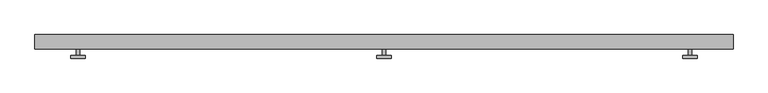
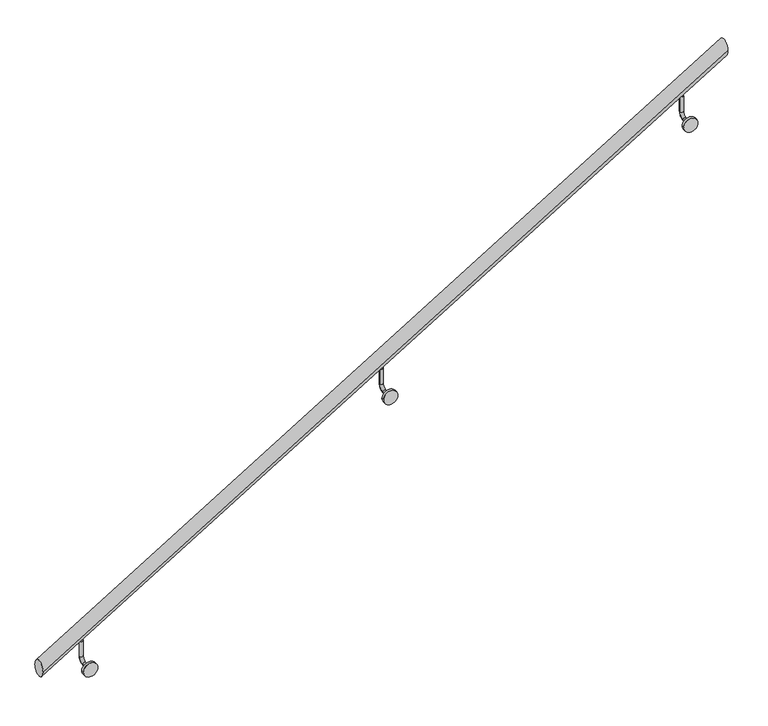
"""IFC4 building model written with IfcOpenShell, lengths in millimetres: railing geometry."""

import ifcopenshell
import ifcopenshell.guid

model = None  # the IFC model being written
_history = None  # IfcOwnerHistory: only IFC2X3 demands one
_inside = {}  # id of a spatial element -> (the spatial element, [elements in it])
_under = {}  # id of a project, library or spatial element -> (it, [spatial elements below it])
_declared = {}  # id of a project -> (the project, [libraries it declares])
_typed = {}  # id of a type object -> (the type object, [elements of that type])
_made_of = {}  # id of a material, layer set ... -> (it, [elements and type objects made of it])


def new_model(schema):
    """Start an empty IFC model of exactly this schema.

    Asked for "IFC4X3", IfcOpenShell would pick the latest addendum, in which some entities
    have other attributes; the version numbers below select the first issue.
    IFC2X3 requires an IfcOwnerHistory on every rooted entity: one is made here for all.
    """
    global model, _history
    if schema == "IFC4X3":
        model = ifcopenshell.file(schema_version=(4, 3, 0, 0))
    else:
        model = ifcopenshell.file(schema=schema)
    _inside.clear()
    _under.clear()
    _declared.clear()
    _typed.clear()
    _made_of.clear()
    _history = None
    if model.schema == "IFC2X3":
        org = make("IfcOrganization", Name="unknown")
        user = make(
            "IfcPersonAndOrganization",
            ThePerson=make("IfcPerson", FamilyName="unknown"),
            TheOrganization=org,
        )
        app = make(
            "IfcApplication",
            ApplicationDeveloper=org,
            Version="unknown",
            ApplicationFullName="unknown",
            ApplicationIdentifier="unknown",
        )
        _history = make(
            "IfcOwnerHistory",
            OwningUser=user,
            OwningApplication=app,
            ChangeAction="ADDED",
            CreationDate=0,
        )
    return model


def make(cls, **values):
    """One entity of the class cls with the attributes given. An attribute that is None is left unset."""
    return model.create_entity(
        cls, **{name: value for name, value in values.items() if value is not None}
    )


def rooted(cls, **values):
    """An entity with a GlobalId (a new one), such as an element, a storey or a relation."""
    return make(cls, GlobalId=ifcopenshell.guid.new(), OwnerHistory=_history, **values)


def si_unit(unit_type, name, prefix=None):
    """IfcSIUnit, for example si_unit("LENGTHUNIT", "METRE", prefix="MILLI")."""
    return make("IfcSIUnit", UnitType=unit_type, Prefix=prefix, Name=name)


def assignment(units):
    """IfcUnitAssignment: the units of a project."""
    return None if units is None else make("IfcUnitAssignment", Units=units)


def point(xyz):
    """IfcCartesianPoint."""
    return None if xyz is None else make("IfcCartesianPoint", Coordinates=xyz)


def direction(xyz):
    """IfcDirection."""
    return None if xyz is None else make("IfcDirection", DirectionRatios=xyz)


def frame(location, z_axis=None, x_axis=None):
    """IfcAxis2Placement3D, a coordinate frame: its origin and axes. An axis left out is left unset."""
    return make(
        "IfcAxis2Placement3D",
        Location=point(location),
        Axis=direction(z_axis),
        RefDirection=direction(x_axis),
    )


def frame_2d(location, x_axis=None):
    """IfcAxis2Placement2D, a coordinate frame in the plane: its origin and x axis."""
    return make(
        "IfcAxis2Placement2D", Location=point(location), RefDirection=direction(x_axis)
    )


def origin():
    """The frame at (0, 0, 0) with its axes left unset."""
    return frame((0.0, 0.0, 0.0))


def place(relative_to, where):
    """IfcLocalPlacement: puts the frame where relative to a parent placement (None: the world)."""
    return make(
        "IfcLocalPlacement", PlacementRelTo=relative_to, RelativePlacement=where
    )


def context(
    kind, dimensions, precision=None, world=None, true_north=None, identifier=None
):
    """IfcGeometricRepresentationContext, for example the 3D "Model" context."""
    return make(
        "IfcGeometricRepresentationContext",
        ContextIdentifier=identifier,
        ContextType=kind,
        CoordinateSpaceDimension=dimensions,
        Precision=precision,
        WorldCoordinateSystem=world,
        TrueNorth=true_north,
    )


def project(units=None, contexts=None):
    """IfcProject with its units and contexts."""
    return rooted(
        "IfcProject",
        Name="project",
        RepresentationContexts=contexts,
        UnitsInContext=assignment(units),
    )


def spatial(cls, under=None, at=None, **own):
    """A site, building, storey or space (cls), placed at a placement, below another one or the project."""
    s = rooted(cls, ObjectPlacement=at, **own)
    if under is not None:
        _under.setdefault(under.id(), (under, []))[1].append(s)
    return s


def circle_curve(where, radius):
    """IfcCircle in the frame where."""
    return make("IfcCircle", Position=where, Radius=radius)


def ellipse_curve(where, semi_axis1, semi_axis2):
    """IfcEllipse in the frame where."""
    return make(
        "IfcEllipse", Position=where, SemiAxis1=semi_axis1, SemiAxis2=semi_axis2
    )


def trimmed(basis, trim1, trim2, sense, master):
    """IfcTrimmedCurve: the piece of a basis curve between two trims."""
    return make(
        "IfcTrimmedCurve",
        BasisCurve=basis,
        Trim1=trim1,
        Trim2=trim2,
        SenseAgreement=sense,
        MasterRepresentation=master,
    )


def segment(curve, same_sense, transition):
    """IfcCompositeCurveSegment."""
    return make(
        "IfcCompositeCurveSegment",
        Transition=transition,
        SameSense=same_sense,
        ParentCurve=curve,
    )


def composite_curve(segments, self_intersect=None):
    """IfcCompositeCurve: segments joined end to end."""
    return make("IfcCompositeCurve", Segments=segments, SelfIntersect=self_intersect)


def outline(outer, holes=None, kind="AREA"):
    """IfcArbitraryClosedProfileDef: a profile drawn as a closed curve; with holes, ...WithVoids."""
    if holes is None:
        return make("IfcArbitraryClosedProfileDef", ProfileType=kind, OuterCurve=outer)
    return make(
        "IfcArbitraryProfileDefWithVoids",
        ProfileType=kind,
        OuterCurve=outer,
        InnerCurves=holes,
    )


def extrude(swept, where, along, depth):
    """IfcExtrudedAreaSolid: the profile swept, set in the frame where, extruded along a direction by depth."""
    return make(
        "IfcExtrudedAreaSolid",
        SweptArea=swept,
        Position=where,
        ExtrudedDirection=direction(along),
        Depth=depth,
    )


def shape(context_of_items, identifier, shape_type, items):
    """IfcShapeRepresentation: the items that make up one representation, for example the "Body"."""
    return make(
        "IfcShapeRepresentation",
        ContextOfItems=context_of_items,
        RepresentationIdentifier=identifier,
        RepresentationType=shape_type,
        Items=items,
    )


def source(mapping_origin, context_of_items, identifier, shape_type, items):
    """IfcRepresentationMap: a shape defined once, which mapped items show again and again."""
    return make(
        "IfcRepresentationMap",
        MappingOrigin=mapping_origin,
        MappedRepresentation=shape(context_of_items, identifier, shape_type, items),
    )


def transform(
    local_origin,
    x_axis=None,
    y_axis=None,
    z_axis=None,
    scale=None,
    scale2=None,
    scale3=None,
    uniform=True,
):
    """IfcCartesianTransformationOperator3D, or its non-uniform kind. x_axis, y_axis, z_axis: its Axis1, 2, 3."""
    if uniform:
        return make(
            "IfcCartesianTransformationOperator3D",
            Axis1=direction(x_axis),
            Axis2=direction(y_axis),
            LocalOrigin=point(local_origin),
            Scale=scale,
            Axis3=direction(z_axis),
        )
    return make(
        "IfcCartesianTransformationOperator3DnonUniform",
        Axis1=direction(x_axis),
        Axis2=direction(y_axis),
        LocalOrigin=point(local_origin),
        Scale=scale,
        Axis3=direction(z_axis),
        Scale2=scale2,
        Scale3=scale3,
    )


def mapped(mapping_source, mapping_target):
    """IfcMappedItem: shows the shape of a source again, moved by a transform."""
    return make(
        "IfcMappedItem", MappingSource=mapping_source, MappingTarget=mapping_target
    )


def made_of(thing, what):
    """Note that an element or type object is made of a material, layer set ...; save() writes the relation."""
    if what is not None:
        _made_of.setdefault(what.id(), (what, []))[1].append(thing)
    return thing


def element(
    cls,
    number,
    at=None,
    inside=None,
    cuts=None,
    type_object=None,
    material=None,
    context=None,
    identifier="Body",
    shape_type=None,
    held_by="IfcProductDefinitionShape",
    body=None,
    shapes=None,
    **own,
):
    """One element of the class cls, such as IfcWall. Its Tag is "e" and its number.

    at: its placement. inside: the storey or other place that contains it. cuts: it is an
    opening in that element (IfcRelVoidsElement). A single representation is given by context,
    identifier, shape_type and body (its items); several are given by shapes. held_by: the class
    of the entity that holds the representations. save() writes the other relations.
    """
    e = rooted(cls, Tag="e%d" % number, ObjectPlacement=at, **own)
    if body is not None:
        shapes = [shape(context, identifier, shape_type, body)]
    if shapes is not None:
        e.Representation = make(held_by, Representations=shapes)
    if inside is not None:
        _inside.setdefault(inside.id(), (inside, []))[1].append(e)
    if cuts is not None:
        rooted(
            "IfcRelVoidsElement", RelatingBuildingElement=cuts, RelatedOpeningElement=e
        )
    if type_object is not None:
        _typed.setdefault(type_object.id(), (type_object, []))[1].append(e)
    return made_of(e, material)


def aggregate(whole, parts):
    """IfcRelAggregates: a whole, such as a stair, and the parts it consists of."""
    return rooted("IfcRelAggregates", RelatingObject=whole, RelatedObjects=parts)


def save(model, path):
    """Write the relations noted so far, then the file.

    IfcRelAggregates (storeys below a building ...), IfcRelContainedInSpatialStructure (elements
    in a storey), IfcRelDefinesByType, IfcRelAssociatesMaterial and IfcRelDeclares: one each for
    every whole, place, type object, material and project.
    """
    for whole, parts in _under.values():
        aggregate(whole, parts)
    for where, things in _inside.values():
        rooted(
            "IfcRelContainedInSpatialStructure",
            RelatedElements=things,
            RelatingStructure=where,
        )
    for kind, things in _typed.values():
        rooted("IfcRelDefinesByType", RelatedObjects=things, RelatingType=kind)
    for what, things in _made_of.values():
        rooted("IfcRelAssociatesMaterial", RelatedObjects=things, RelatingMaterial=what)
    for by, libraries in _declared.values():
        rooted("IfcRelDeclares", RelatingContext=by, RelatedDefinitions=libraries)
    model.write(path)


def plane_surface(at):
    """IfcPlane: the flat surface through the origin of the frame at, square to its z axis."""
    return make("IfcPlane", Position=at)


def cylinder_surface(at, radius):
    """IfcCylindricalSurface: all points at the distance radius from the z axis of the frame at."""
    return make("IfcCylindricalSurface", Position=at, Radius=radius)


def revolved_surface(curve, axis_point, axis_direction):
    """IfcSurfaceOfRevolution: the curve turned about the line through axis_point along axis_direction."""
    return make(
        "IfcSurfaceOfRevolution",
        SweptCurve=make("IfcArbitraryOpenProfileDef", ProfileType="CURVE", Curve=curve),
        AxisPosition=make("IfcAxis1Placement", Location=point(axis_point), Axis=direction(axis_direction)),
    )


def advanced_brep(points, edges, surfaces, faces):
    """IfcAdvancedBrep: a solid bounded by faces that lie on surfaces and meet in shared edges.

    An edge is (start, end): straight between two places in points (the first is 0);
    or (start, end, curve); or (start, end, curve, False) where it runs against its curve.
    A face is (place in surfaces, loops), or (place, loops, False) where it looks against
    its surface's normal. A loop lists edges by number (the first is 1), with a minus sign
    where the edge is run from its end to its start. The first loop is the outer one.
    """
    corners = [point(p) for p in points]
    vertices = [make("IfcVertexPoint", VertexGeometry=c) for c in corners]
    made = []
    for start, end, *more in edges:
        made.append(
            make(
                "IfcEdgeCurve",
                EdgeStart=vertices[start],
                EdgeEnd=vertices[end],
                EdgeGeometry=more[0] if more else make("IfcPolyline", Points=[corners[start], corners[end]]),
                SameSense=more[1] if len(more) > 1 else True,
            )
        )
    hull = []
    for where, loops, *sense in faces:
        bounds = []
        for j, loop in enumerate(loops):
            ring = [make("IfcOrientedEdge", EdgeElement=made[abs(k) - 1], Orientation=k > 0) for k in loop]
            bounds.append(
                make(
                    "IfcFaceOuterBound" if j == 0 else "IfcFaceBound",
                    Bound=make("IfcEdgeLoop", EdgeList=ring),
                    Orientation=True,
                )
            )
        hull.append(make("IfcAdvancedFace", Bounds=bounds, FaceSurface=surfaces[where], SameSense=sense[0] if sense else True))
    return make("IfcAdvancedBrep", Outer=make("IfcClosedShell", CfsFaces=hull))


def railing_5f4a1c35(model_context):
    return source(origin(), model_context, "Body", "SolidModel", [
        advanced_brep(
        [(-50191.7895023, 15484.3574868, 6395.7778144), (-50191.7895023, 15434.3574868, 6395.7778144), (-47761.7895023, 15484.3574868, 7876.1226419), (-47761.7895023, 15434.3574868, 7876.1226419)],
        [
            (0, 1, ellipse_curve(frame((-50191.7895023, 15459.3574868, 6395.7778144), z_axis=(-1.0, 0.0, 0.0), x_axis=(0.0, 0.0, -1.0)), 29.2736981, 25.0)),
            (1, 0, ellipse_curve(frame((-50191.7895023, 15459.3574868, 6395.7778144), z_axis=(-1.0, 0.0, 0.0), x_axis=(0.0, 0.0, -1.0)), 29.2736981, 25.0)),
            (2, 3, ellipse_curve(frame((-47761.7895023, 15459.3574868, 7876.1226419), z_axis=(1.0, 0.0, 0.0), x_axis=(0.0, 0.0, -1.0)), 29.2736981, 25.0)),
            (3, 2, ellipse_curve(frame((-47761.7895023, 15459.3574868, 7876.1226419), z_axis=(1.0, 0.0, 0.0), x_axis=(0.0, 0.0, -1.0)), 29.2736981, 25.0)),
            (0, 2),
            (3, 1),
        ],
        [
            plane_surface(frame((-50191.7895023, 15459.3574868, 6425.0515124), z_axis=(-1.0, 0.0, 0.0), x_axis=(0.0, 1.0, 0.0))),
            plane_surface(frame((-47761.7895023, 15459.3574868, 7905.39634), z_axis=(1.0, 0.0, 0.0), x_axis=(0.0, 1.0, 0.0))),
            cylinder_surface(frame((-50178.7830443, 15459.3574868, 6403.7012888), z_axis=(-0.8540089447440432, 0.0, -0.5202583226601627), x_axis=(0.0, -1.0, 0.0)), 25.0),
        ],
        [
            (0, [[1, 2]]),
            (1, [[3, 4]]),
            (2, [[-1, 5, -4, 6]]),
            (2, [[-2, -6, -3, -5]]),
        ],
    ),
        advanced_brep(
        [(-48983.1395023, 15459.3574868, 7096.1739262), (-48970.4395023, 15459.3574868, 7096.1739262), (-48983.1395023, 15459.3574868, 7039.0239262), (-48970.4395023, 15459.3574868, 7039.0239262), (-48970.4395023, 15440.3074868, 7019.9739262), (-48983.1395023, 15440.3074868, 7019.9739262), (-48983.1395023, 15411.7324868, 7019.9739262), (-48970.4395023, 15411.7324868, 7019.9739262)],
        [
            (0, 1, circle_curve(frame((-48976.7895023, 15459.3574868, 7096.1739262), z_axis=(0.0, 0.0, 1.0), x_axis=(1.0, 0.0, 0.0)), 6.35)),
            (1, 0, circle_curve(frame((-48976.7895023, 15459.3574868, 7096.1739262), z_axis=(0.0, 0.0, 1.0), x_axis=(1.0, 0.0, 0.0)), 6.35)),
            (0, 2),
            (2, 3, circle_curve(frame((-48976.7895023, 15459.3574868, 7039.0239262), z_axis=(0.0, 0.0, 1.0), x_axis=(1.0, 0.0, 0.0)), 6.35)),
            (3, 1),
            (3, 2, circle_curve(frame((-48976.7895023, 15459.3574868, 7039.0239262), z_axis=(0.0, 0.0, 1.0), x_axis=(1.0, 0.0, 0.0)), 6.35)),
            (4, 3, circle_curve(frame((-48970.4395023, 15440.3074868, 7039.0239262), z_axis=(1.0, 0.0, 0.0), x_axis=(0.0, 1.0, 0.0)), 19.05)),
            (2, 5, circle_curve(frame((-48983.1395023, 15440.3074868, 7039.0239262), z_axis=(-1.0, 0.0, 0.0), x_axis=(0.0, 1.0, 0.0)), 19.05)),
            (5, 4, circle_curve(frame((-48976.7895023, 15440.3074868, 7019.9739262), z_axis=(0.0, 1.0, 0.0), x_axis=(1.0, 0.0, 0.0)), 6.35)),
            (4, 5, circle_curve(frame((-48976.7895023, 15440.3074868, 7019.9739262), z_axis=(0.0, 1.0, 0.0), x_axis=(1.0, 0.0, 0.0)), 6.35)),
            (6, 7, circle_curve(frame((-48976.7895023, 15411.7324868, 7019.9739262), z_axis=(0.0, -1.0, 0.0), x_axis=(1.0, 0.0, 0.0)), 6.35)),
            (7, 6, circle_curve(frame((-48976.7895023, 15411.7324868, 7019.9739262), z_axis=(0.0, -1.0, 0.0), x_axis=(1.0, 0.0, 0.0)), 6.35)),
            (5, 6),
            (7, 4),
        ],
        [
            plane_surface(frame((-48970.4395023, 15459.3574868, 7096.1739262), z_axis=(0.0, 0.0, 1.0), x_axis=(0.0, -1.0, 0.0))),
            cylinder_surface(frame((-48976.7895023, 15459.3574868, 7096.1739262), z_axis=(0.0, 0.0, 1.0), x_axis=(1.0, 0.0, 0.0)), 6.35),
            revolved_surface(trimmed(ellipse_curve(frame((-48976.7895023, 15459.3574868, 7039.0239262), z_axis=(0.0, 0.0, 1.0), x_axis=(1.0, 0.0, 0.0)), 6.35, 6.35), [point((-48983.1395023, 15459.3574868, 7039.0239262))], [point((-48970.4395023, 15459.3574868, 7039.0239262))], True, "CARTESIAN"), (-48976.7895023, 15440.3074868, 7039.0239262), (-1.0, 0.0, 0.0)),
            revolved_surface(trimmed(ellipse_curve(frame((-48976.7895023, 15459.3574868, 7039.0239262), z_axis=(0.0, 0.0, 1.0), x_axis=(1.0, 0.0, 0.0)), 6.35, 6.35), [point((-48970.4395023, 15459.3574868, 7039.0239262))], [point((-48983.1395023, 15459.3574868, 7039.0239262))], True, "CARTESIAN"), (-48976.7895023, 15440.3074868, 7039.0239262), (-1.0, 0.0, 0.0)),
            plane_surface(frame((-48976.7895023, 15411.7324868, 7013.6239262), z_axis=(0.0, -1.0, 0.0), x_axis=(1.0, 0.0, 0.0))),
            cylinder_surface(frame((-48976.7895023, 15440.3074868, 7019.9739262), z_axis=(0.0, 1.0, 0.0), x_axis=(1.0, 0.0, 0.0)), 6.35),
        ],
        [
            (0, [[1, 2]]),
            (1, [[-1, 3, 4, 5]]),
            (1, [[-2, -5, 6, -3]]),
            (2, [[7, -4, 8, 9]]),
            (3, [[-8, -6, -7, 10]]),
            (4, [[11, 12]]),
            (5, [[-9, 13, -12, 14]]),
            (5, [[-10, -14, -11, -13]]),
        ],
    ),
        extrude(outline(composite_curve([segment(trimmed(circle_curve(frame_2d((7019.9739262, -48976.7895023)), 25.4), [point((7019.9739262, -48951.3895023))], [point((7019.9739262, -49002.1895023))], False, "CARTESIAN"), True, "CONTINUOUS"), segment(trimmed(circle_curve(frame_2d((7019.9739262, -48976.7895023)), 25.4), [point((7019.9739262, -49002.1895023))], [point((7019.9739262, -48951.3895023))], False, "CARTESIAN"), True, "CONTINUOUS")], self_intersect=False)), frame((0.0, 15402.2074868, 0.0), z_axis=(0.0, 1.0, 0.0), x_axis=(0.0, 0.0, 1.0)), (0.0, 0.0, 1.0), 9.525),
        advanced_brep(
        [(-47918.1395023, 15459.3574868, 7744.9670297), (-47905.4395023, 15459.3574868, 7744.9670297), (-47918.1395023, 15459.3574868, 7687.8170297), (-47905.4395023, 15459.3574868, 7687.8170297), (-47905.4395023, 15440.3074868, 7668.7670297), (-47918.1395023, 15440.3074868, 7668.7670297), (-47918.1395023, 15411.7324868, 7668.7670297), (-47905.4395023, 15411.7324868, 7668.7670297)],
        [
            (0, 1, circle_curve(frame((-47911.7895023, 15459.3574868, 7744.9670297), z_axis=(0.0, 0.0, 1.0), x_axis=(1.0, 0.0, 0.0)), 6.35)),
            (1, 0, circle_curve(frame((-47911.7895023, 15459.3574868, 7744.9670297), z_axis=(0.0, 0.0, 1.0), x_axis=(1.0, 0.0, 0.0)), 6.35)),
            (0, 2),
            (2, 3, circle_curve(frame((-47911.7895023, 15459.3574868, 7687.8170297), z_axis=(0.0, 0.0, 1.0), x_axis=(1.0, 0.0, 0.0)), 6.35)),
            (3, 1),
            (3, 2, circle_curve(frame((-47911.7895023, 15459.3574868, 7687.8170297), z_axis=(0.0, 0.0, 1.0), x_axis=(1.0, 0.0, 0.0)), 6.35)),
            (4, 3, circle_curve(frame((-47905.4395023, 15440.3074868, 7687.8170297), z_axis=(1.0, 0.0, 0.0), x_axis=(0.0, 1.0, 0.0)), 19.05)),
            (2, 5, circle_curve(frame((-47918.1395023, 15440.3074868, 7687.8170297), z_axis=(-1.0, 0.0, 0.0), x_axis=(0.0, 1.0, 0.0)), 19.05)),
            (5, 4, circle_curve(frame((-47911.7895023, 15440.3074868, 7668.7670297), z_axis=(0.0, 1.0, 0.0), x_axis=(1.0, 0.0, 0.0)), 6.35)),
            (4, 5, circle_curve(frame((-47911.7895023, 15440.3074868, 7668.7670297), z_axis=(0.0, 1.0, 0.0), x_axis=(1.0, 0.0, 0.0)), 6.35)),
            (6, 7, circle_curve(frame((-47911.7895023, 15411.7324868, 7668.7670297), z_axis=(0.0, -1.0, 0.0), x_axis=(1.0, 0.0, 0.0)), 6.35)),
            (7, 6, circle_curve(frame((-47911.7895023, 15411.7324868, 7668.7670297), z_axis=(0.0, -1.0, 0.0), x_axis=(1.0, 0.0, 0.0)), 6.35)),
            (5, 6),
            (7, 4),
        ],
        [
            plane_surface(frame((-47905.4395023, 15459.3574868, 7744.9670297), z_axis=(0.0, 0.0, 1.0), x_axis=(0.0, -1.0, 0.0))),
            cylinder_surface(frame((-47911.7895023, 15459.3574868, 7744.9670297), z_axis=(0.0, 0.0, 1.0), x_axis=(1.0, 0.0, 0.0)), 6.35),
            revolved_surface(trimmed(ellipse_curve(frame((-47911.7895023, 15459.3574868, 7687.8170297), z_axis=(0.0, 0.0, 1.0), x_axis=(1.0, 0.0, 0.0)), 6.35, 6.35), [point((-47918.1395023, 15459.3574868, 7687.8170297))], [point((-47905.4395023, 15459.3574868, 7687.8170297))], True, "CARTESIAN"), (-47911.7895023, 15440.3074868, 7687.8170297), (-1.0, 0.0, 0.0)),
            revolved_surface(trimmed(ellipse_curve(frame((-47911.7895023, 15459.3574868, 7687.8170297), z_axis=(0.0, 0.0, 1.0), x_axis=(1.0, 0.0, 0.0)), 6.35, 6.35), [point((-47905.4395023, 15459.3574868, 7687.8170297))], [point((-47918.1395023, 15459.3574868, 7687.8170297))], True, "CARTESIAN"), (-47911.7895023, 15440.3074868, 7687.8170297), (-1.0, 0.0, 0.0)),
            plane_surface(frame((-47911.7895023, 15411.7324868, 7662.4170297), z_axis=(0.0, -1.0, 0.0), x_axis=(1.0, 0.0, 0.0))),
            cylinder_surface(frame((-47911.7895023, 15440.3074868, 7668.7670297), z_axis=(0.0, 1.0, 0.0), x_axis=(1.0, 0.0, 0.0)), 6.35),
        ],
        [
            (0, [[1, 2]]),
            (1, [[-1, 3, 4, 5]]),
            (1, [[-2, -5, 6, -3]]),
            (2, [[7, -4, 8, 9]]),
            (3, [[-8, -6, -7, 10]]),
            (4, [[11, 12]]),
            (5, [[-9, 13, -12, 14]]),
            (5, [[-10, -14, -11, -13]]),
        ],
    ),
        extrude(outline(composite_curve([segment(trimmed(circle_curve(frame_2d((7668.7670297, -47911.7895023)), 25.4), [point((7668.7670297, -47886.3895023))], [point((7668.7670297, -47937.1895023))], False, "CARTESIAN"), True, "CONTINUOUS"), segment(trimmed(circle_curve(frame_2d((7668.7670297, -47911.7895023)), 25.4), [point((7668.7670297, -47937.1895023))], [point((7668.7670297, -47886.3895023))], False, "CARTESIAN"), True, "CONTINUOUS")], self_intersect=False)), frame((0.0, 15402.2074868, 0.0), z_axis=(0.0, 1.0, 0.0), x_axis=(0.0, 0.0, 1.0)), (0.0, 0.0, 1.0), 9.525),
        advanced_brep(
        [(-50048.1395023, 15459.3574868, 6447.3808228), (-50035.4395023, 15459.3574868, 6447.3808228), (-50048.1395023, 15459.3574868, 6390.2308228), (-50035.4395023, 15459.3574868, 6390.2308228), (-50035.4395023, 15440.3074868, 6371.1808228), (-50048.1395023, 15440.3074868, 6371.1808228), (-50048.1395023, 15411.7324868, 6371.1808228), (-50035.4395023, 15411.7324868, 6371.1808228)],
        [
            (0, 1, circle_curve(frame((-50041.7895023, 15459.3574868, 6447.3808228), z_axis=(0.0, 0.0, 1.0), x_axis=(1.0, 0.0, 0.0)), 6.35)),
            (1, 0, circle_curve(frame((-50041.7895023, 15459.3574868, 6447.3808228), z_axis=(0.0, 0.0, 1.0), x_axis=(1.0, 0.0, 0.0)), 6.35)),
            (0, 2),
            (2, 3, circle_curve(frame((-50041.7895023, 15459.3574868, 6390.2308228), z_axis=(0.0, 0.0, 1.0), x_axis=(1.0, 0.0, 0.0)), 6.35)),
            (3, 1),
            (3, 2, circle_curve(frame((-50041.7895023, 15459.3574868, 6390.2308228), z_axis=(0.0, 0.0, 1.0), x_axis=(1.0, 0.0, 0.0)), 6.35)),
            (4, 3, circle_curve(frame((-50035.4395023, 15440.3074868, 6390.2308228), z_axis=(1.0, 0.0, 0.0), x_axis=(0.0, 1.0, 0.0)), 19.05)),
            (2, 5, circle_curve(frame((-50048.1395023, 15440.3074868, 6390.2308228), z_axis=(-1.0, 0.0, 0.0), x_axis=(0.0, 1.0, 0.0)), 19.05)),
            (5, 4, circle_curve(frame((-50041.7895023, 15440.3074868, 6371.1808228), z_axis=(0.0, 1.0, 0.0), x_axis=(1.0, 0.0, 0.0)), 6.35)),
            (4, 5, circle_curve(frame((-50041.7895023, 15440.3074868, 6371.1808228), z_axis=(0.0, 1.0, 0.0), x_axis=(1.0, 0.0, 0.0)), 6.35)),
            (6, 7, circle_curve(frame((-50041.7895023, 15411.7324868, 6371.1808228), z_axis=(0.0, -1.0, 0.0), x_axis=(1.0, 0.0, 0.0)), 6.35)),
            (7, 6, circle_curve(frame((-50041.7895023, 15411.7324868, 6371.1808228), z_axis=(0.0, -1.0, 0.0), x_axis=(1.0, 0.0, 0.0)), 6.35)),
            (5, 6),
            (7, 4),
        ],
        [
            plane_surface(frame((-50035.4395023, 15459.3574868, 6447.3808228), z_axis=(0.0, 0.0, 1.0), x_axis=(0.0, -1.0, 0.0))),
            cylinder_surface(frame((-50041.7895023, 15459.3574868, 6447.3808228), z_axis=(0.0, 0.0, 1.0), x_axis=(1.0, 0.0, 0.0)), 6.35),
            revolved_surface(trimmed(ellipse_curve(frame((-50041.7895023, 15459.3574868, 6390.2308228), z_axis=(0.0, 0.0, 1.0), x_axis=(1.0, 0.0, 0.0)), 6.35, 6.35), [point((-50048.1395023, 15459.3574868, 6390.2308228))], [point((-50035.4395023, 15459.3574868, 6390.2308228))], True, "CARTESIAN"), (-50041.7895023, 15440.3074868, 6390.2308228), (-1.0, 0.0, 0.0)),
            revolved_surface(trimmed(ellipse_curve(frame((-50041.7895023, 15459.3574868, 6390.2308228), z_axis=(0.0, 0.0, 1.0), x_axis=(1.0, 0.0, 0.0)), 6.35, 6.35), [point((-50035.4395023, 15459.3574868, 6390.2308228))], [point((-50048.1395023, 15459.3574868, 6390.2308228))], True, "CARTESIAN"), (-50041.7895023, 15440.3074868, 6390.2308228), (-1.0, 0.0, 0.0)),
            plane_surface(frame((-50041.7895023, 15411.7324868, 6364.8308228), z_axis=(0.0, -1.0, 0.0), x_axis=(1.0, 0.0, 0.0))),
            cylinder_surface(frame((-50041.7895023, 15440.3074868, 6371.1808228), z_axis=(0.0, 1.0, 0.0), x_axis=(1.0, 0.0, 0.0)), 6.35),
        ],
        [
            (0, [[1, 2]]),
            (1, [[-1, 3, 4, 5]]),
            (1, [[-2, -5, 6, -3]]),
            (2, [[7, -4, 8, 9]]),
            (3, [[-8, -6, -7, 10]]),
            (4, [[11, 12]]),
            (5, [[-9, 13, -12, 14]]),
            (5, [[-10, -14, -11, -13]]),
        ],
    ),
        extrude(outline(composite_curve([segment(trimmed(circle_curve(frame_2d((6371.1808228, -50041.7895023)), 25.4), [point((6371.1808228, -50016.3895023))], [point((6371.1808228, -50067.1895023))], False, "CARTESIAN"), True, "CONTINUOUS"), segment(trimmed(circle_curve(frame_2d((6371.1808228, -50041.7895023)), 25.4), [point((6371.1808228, -50067.1895023))], [point((6371.1808228, -50016.3895023))], False, "CARTESIAN"), True, "CONTINUOUS")], self_intersect=False)), frame((0.0, 15402.2074868, 0.0), z_axis=(0.0, 1.0, 0.0), x_axis=(0.0, 0.0, 1.0)), (0.0, 0.0, 1.0), 9.525),
    ])


if __name__ == "__main__":
    model = new_model("IFC4")
    model_context = context("Model", 3, world=origin())
    ifc_project = project(units=[si_unit("LENGTHUNIT", "METRE", prefix="MILLI")], contexts=[model_context])
    site = spatial("IfcSite", under=ifc_project)
    building = spatial("IfcBuilding", under=site)
    placement = place(None, origin())
    railing_shape = railing_5f4a1c35(model_context)
    element("IfcRailing", 1, at=placement, inside=building, context=model_context, shape_type="MappedRepresentation", body=[
        mapped(railing_shape, transform((0.0, 0.0, 0.0), x_axis=(1.0, 0.0, 0.0), y_axis=(0.0, 1.0, 0.0), z_axis=(0.0, 0.0, 1.0))),
    ])
    save(model, "model.ifc")

# Revit data of these elements
# Project information
#   Projekt-Nummer = "Hier die Projektnummer eintragen!"
#   IfcSite GUID = "3DdyCULLv3kQRx$MQ8PThJ"
#   IfcBuilding GUID = "3DdyCULLv3kQRx$MQ8PThG"
#   IfcProject GUID = "3DdyCULLv3kQRx$MQ8PThH"
#   Classification.Facility.Number = "Co_20_15_58"
#   Classification.Facility.Description = "Office complexes"
#   Project Status = "Projektstatus"
#   Project Address = "Geben Sie die Adresse hier ein"
